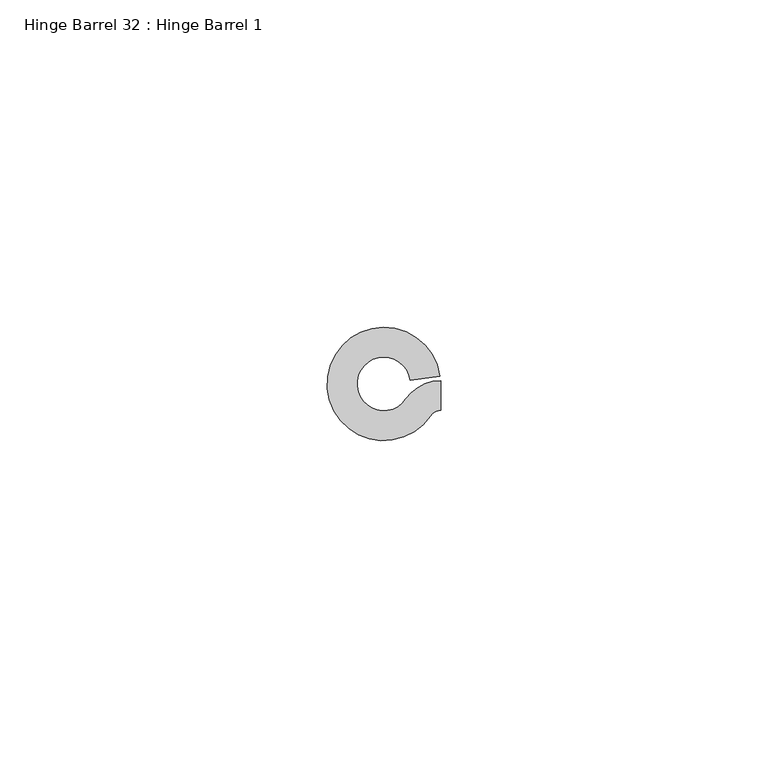
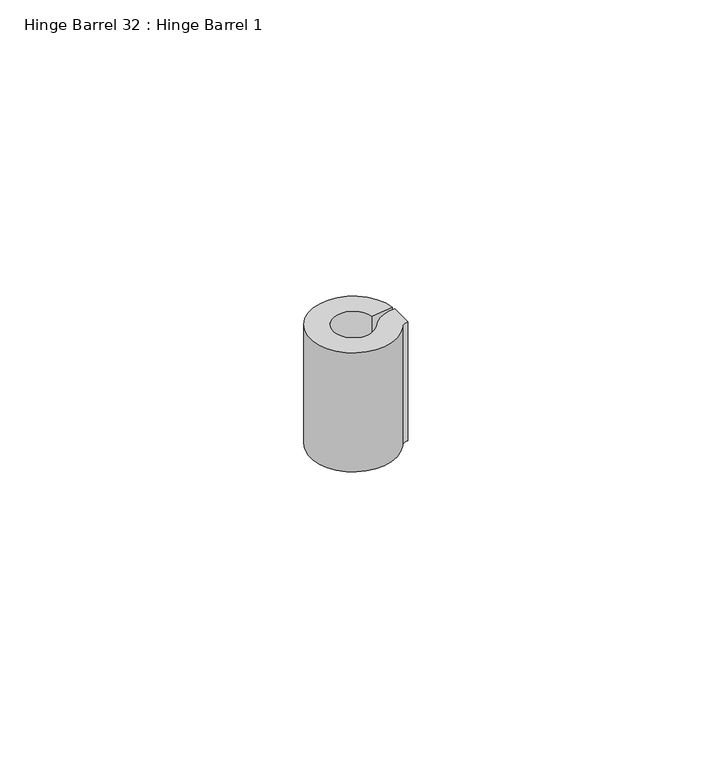
"""IFC4 building model written with IfcOpenShell, lengths in millimetres: proxy geometry, Hinge Barrel 32 : Hinge Barrel 1."""

from ifc_helpers import new_model, si_unit, point, frame, frame_2d, origin, place, context, project, spatial, polyline, circle_curve, trimmed, segment, composite_curve, outline, extrude, source, transform, mapped, element, save


def hinge_barrel_32_hinge_barrel_1_17cad03c(model_context):
    return source(origin(), model_context, "Body", "SweptSolid", [
        extrude(outline(composite_curve([segment(trimmed(circle_curve(frame_2d((587327.8245257, -533990.5568067)), 6.4044851), [point((587322.5194669, -533986.9688017))], [point((587327.8245257, -533984.1523216))], False, "CARTESIAN"), True, "CONTINUOUS"), segment(polyline([(587327.8245257, -533984.1523216), (587327.8245257, -533988.7163841)]), True, "CONTINUOUS"), segment(trimmed(circle_curve(frame_2d((587327.8245257, -533990.5568067)), 1.8404226), [point((587327.8245257, -533988.7163841))], [point((587326.3000393, -533989.5257409))], True, "CARTESIAN"), True, "CONTINUOUS"), segment(trimmed(circle_curve(frame_2d((587319.1320739, -533984.6777841)), 8.6534625), [point((587326.3000393, -533989.5257409))], [point((587327.7022899, -533983.4803654))], False, "CARTESIAN"), True, "CONTINUOUS"), segment(polyline([(587327.7022899, -533983.4803654), (587323.1821338, -533984.1119153)]), True, "CONTINUOUS"), segment(trimmed(circle_curve(frame_2d((587319.1320739, -533984.6777841)), 4.0894), [point((587323.1821338, -533984.1119153))], [point((587322.5194669, -533986.9688017))], True, "CARTESIAN"), True, "CONTINUOUS")], self_intersect=False)), frame((0.0, 0.0, 1149.35), z_axis=(0.0, 0.0, 1.0), x_axis=(1.0, 0.0, 0.0)), (0.0, 0.0, 1.0), 25.4),
    ])


if __name__ == "__main__":
    model = new_model("IFC4")
    model_context = context("Model", 3, world=origin())
    ifc_project = project(units=[si_unit("LENGTHUNIT", "METRE", prefix="MILLI")], contexts=[model_context])
    site = spatial("IfcSite", under=ifc_project)
    building = spatial("IfcBuilding", under=site)
    placement = place(None, origin())
    hinge_barrel_32_hinge_barrel_1_shape = hinge_barrel_32_hinge_barrel_1_17cad03c(model_context)
    element("IfcBuildingElementProxy", 1, Name="Hinge Barrel 32 : Hinge Barrel 1", ObjectType="Hinge Barrel 32 : Hinge Barrel 1", at=placement, inside=building, context=model_context, shape_type="MappedRepresentation", body=[
        mapped(hinge_barrel_32_hinge_barrel_1_shape, transform((0.0, 0.0, 0.0), x_axis=(1.0, 0.0, 0.0), y_axis=(0.0, 1.0, 0.0), z_axis=(0.0, 0.0, 1.0))),
    ])
    save(model, "model.ifc")

# Revit data of these elements
# Element 1 (IfcBuildingElementProxy, "Hinge Barrel 32 : Hinge Barrel 1")
#   Materials on its faces: "6\"X6\" WELD-ON STL BUTT HINGE"
# Materials
#   "6\"X6\" WELD-ON STL BUTT HINGE": class "Metal", colour RGB 189 187 185, transparency 0, Description = "Carbon steel", Cost = 0
